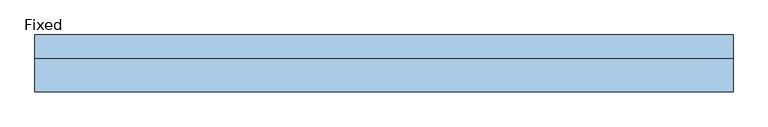
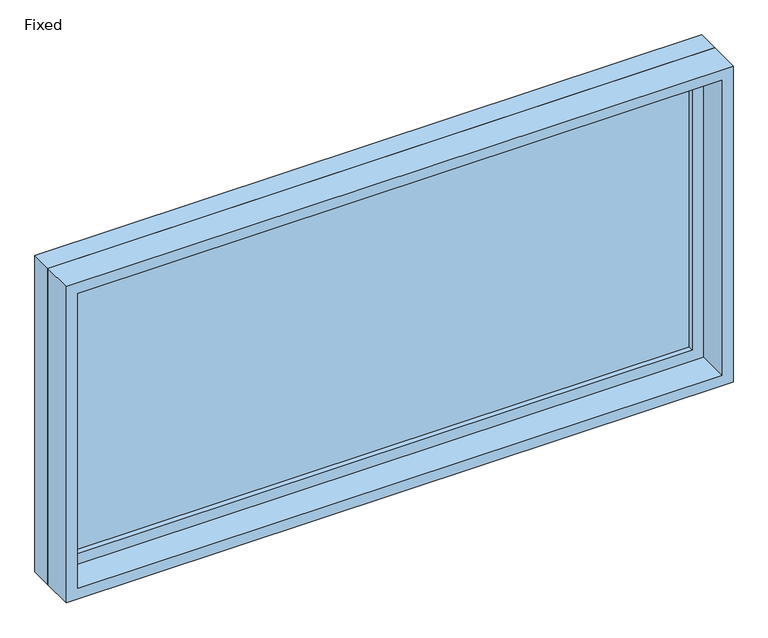
"""IFC4 building model written with IfcOpenShell, lengths in millimetres: window geometry, Fixed."""

from ifc_helpers import new_model, si_unit, frame, origin, place, context, project, spatial, polyline, outline, extrude, source, transform, mapped, element, save


def fixed_992eda32(model_context):
    return source(origin(), model_context, "Body", "SweptSolid", [
        extrude(outline(polyline([(835.025, 28.575), (-911.225, 28.575), (-911.225, 41.275), (835.025, 41.275), (835.025, 28.575)])), frame((0.0, 0.0, 1257.3), z_axis=(0.0, 0.0, 1.0), x_axis=(1.0, 0.0, 0.0)), (0.0, 0.0, 1.0), 812.8),
        extrude(outline(polyline([(2114.55, -955.675), (1212.85, -955.675), (1212.85, 879.475), (2114.55, 879.475), (2114.55, -955.675)]), holes=[polyline([(2070.1, -911.225), (2070.1, 835.025), (1257.3, 835.025), (1257.3, -911.225), (2070.1, -911.225)])]), frame((0.0, 12.7, 0.0), z_axis=(0.0, 1.0, 0.0), x_axis=(0.0, 0.0, 1.0)), (0.0, 0.0, 1.0), 44.45),
        extrude(outline(polyline([(2133.6, -974.725), (1193.8, -974.725), (1193.8, 898.525), (2133.6, 898.525), (2133.6, -974.725)]), holes=[polyline([(2101.85, -942.975), (2101.85, 866.775), (1225.55, 866.775), (1225.55, -942.975), (2101.85, -942.975)])]), frame((0.0, -76.2, 0.0), z_axis=(0.0, 1.0, 0.0), x_axis=(0.0, 0.0, 1.0)), (0.0, 0.0, 1.0), 88.9),
        extrude(outline(polyline([(2133.6, 898.525), (2133.6, -974.725), (1193.8, -974.725), (1193.8, 898.525), (2133.6, 898.525)]), holes=[polyline([(2114.55, 879.475), (1212.85, 879.475), (1212.85, -955.675), (2114.55, -955.675), (2114.55, 879.475)])]), frame((0.0, 12.7, 0.0), z_axis=(0.0, 1.0, 0.0), x_axis=(0.0, 0.0, 1.0)), (0.0, 0.0, 1.0), 63.5),
    ])


if __name__ == "__main__":
    model = new_model("IFC4")
    model_context = context("Model", 3, world=origin())
    ifc_project = project(units=[si_unit("LENGTHUNIT", "METRE", prefix="MILLI")], contexts=[model_context])
    site = spatial("IfcSite", under=ifc_project)
    building = spatial("IfcBuilding", under=site)
    placement = place(None, origin())
    fixed_shape = fixed_992eda32(model_context)
    element("IfcWindow", 1, ObjectType="Fixed : 6' 1 34\"\" x 3' 1\"", at=placement, inside=building, context=model_context, shape_type="MappedRepresentation", body=[
        mapped(fixed_shape, transform((0.0, 0.0, 0.0), x_axis=(1.0, 0.0, 0.0), y_axis=(0.0, 1.0, 0.0), z_axis=(0.0, 0.0, 1.0))),
    ])
    save(model, "model.ifc")

# Revit data of these elements
# Type "Fixed : 6' 1 34\"\" x 3' 1\""
#   Type Mark = "10"
#   Assembly Code = "B2020100"
#   Height = 3' - 1"
#   Default Sill Height = 3' - 11"
#   Width = 6' - 1 3/4"
#   Window Inset = 0' - 0 3/4"
#   Glass Pane Material = Glass
#   Sash Material = Sash
#   Wall Closure = (empty or 0)
# Element 1 (IfcWindow, "Fixed : 6' 1 34\"\" x 3' 1\"")
#   Materials on its faces: "Sash", "Glass"
# Materials
#   "Glass": class "Glass", colour RGB 218 227 224, transparency 0.85, Description = "Soda Lime Glass", Cost = 0
#   "Sash": class "Wood", colour RGB 136 99 55, transparency 0
